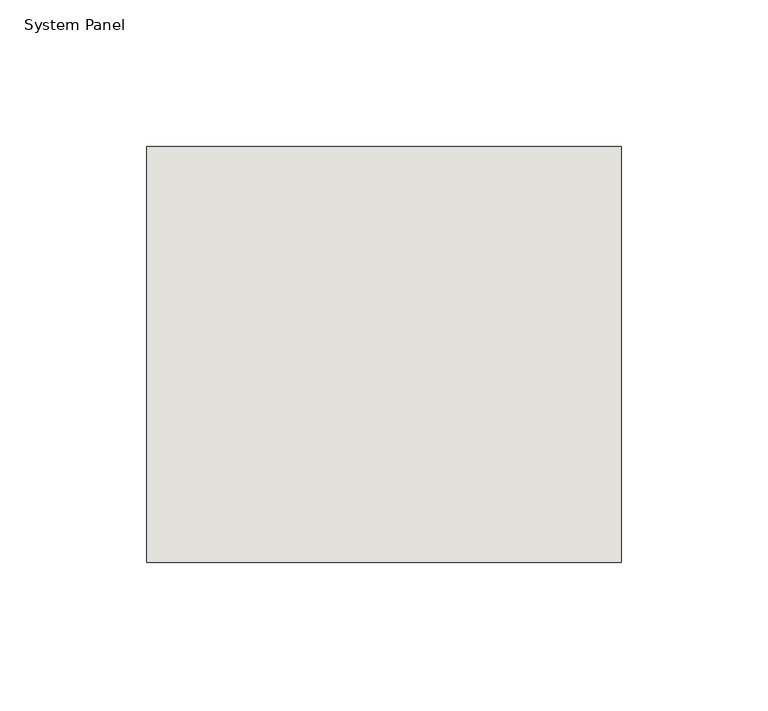
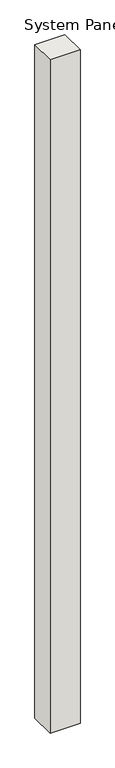
"""IFC4 building model written with IfcOpenShell, lengths in millimetres: wall geometry, System Panel : NLRS_21_CWP_hsb-vulling minerale wol 142 _gen_rsf."""

from ifc_helpers import new_model, si_unit, origin, origin_with_axes, place, context, project, spatial, polyline, outline, extrude, source, transform, mapped, element, save


def system_panel_9935ab3f(model_context):
    return source(origin(), model_context, "Body", "SweptSolid", [
        extrude(outline(polyline([(80.9999998, -71.0), (-80.9999998, -71.0), (-80.9999998, 71.0), (80.9999998, 71.0), (80.9999998, -71.0)])), origin_with_axes(), (0.0, 0.0, 1.0), 3849.0),
    ])


if __name__ == "__main__":
    model = new_model("IFC4")
    model_context = context("Model", 3, world=origin())
    ifc_project = project(units=[si_unit("LENGTHUNIT", "METRE", prefix="MILLI")], contexts=[model_context])
    site = spatial("IfcSite", under=ifc_project)
    building = spatial("IfcBuilding", under=site)
    placement = place(None, origin())
    system_panel_shape = system_panel_9935ab3f(model_context)
    element("IfcWall", 1, ObjectType="System Panel : NLRS_21_CWP_hsb-vulling minerale wol 142 _gen_rsf", at=placement, inside=building, context=model_context, shape_type="MappedRepresentation", body=[
        mapped(system_panel_shape, transform((0.0, 0.0, 0.0), x_axis=(1.0, 0.0, 0.0), y_axis=(0.0, 1.0, 0.0), z_axis=(0.0, 0.0, 1.0))),
    ])
    save(model, "model.ifc")

# Revit data of these elements
# Type "System Panel : NLRS_21_CWP_hsb-vulling minerale wol 142 _gen_rsf"
#   Type IfcGUID = "07M7mRoiH1CR8m_RSKIwpC"
#   Assembly Code = "21.23"
#   IfcExportAs = "IfcWall"
# Element 1 (IfcWall, "System Panel : NLRS_21_CWP_hsb-vulling minerale wol 142 _gen_rsf")
#   Materials on its faces: "NLRS_m1_isolatie minerale wol_gen_rsf"
# Materials
#   "NLRS_m1_isolatie minerale wol_gen_rsf": class "M - Anorganische materialen", colour RGB 200 200 140, transparency 0, Keynote = "m1", Manufacturer = "Revit Standards Foundation", URL = "www.revitstandards.org", Description = "isolatie minerale wol", Cost = 0
